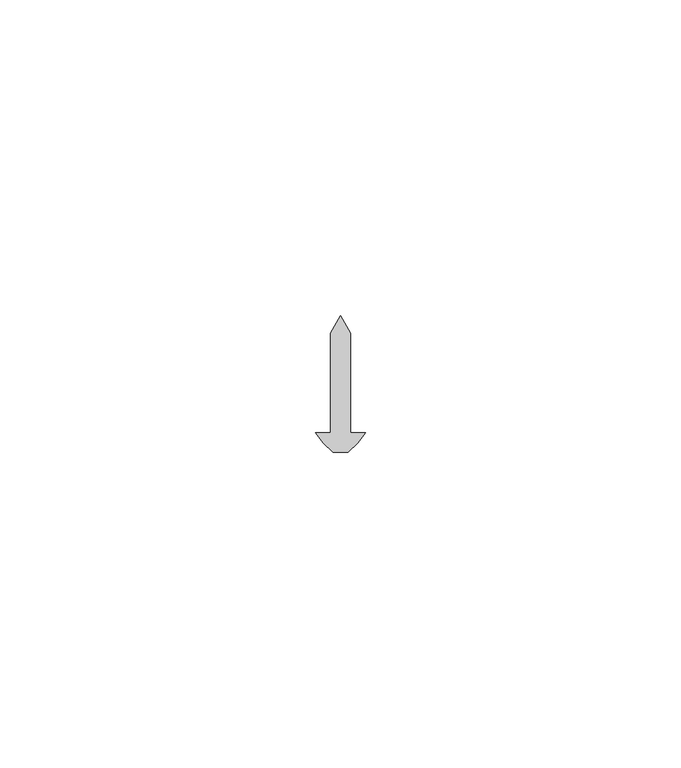
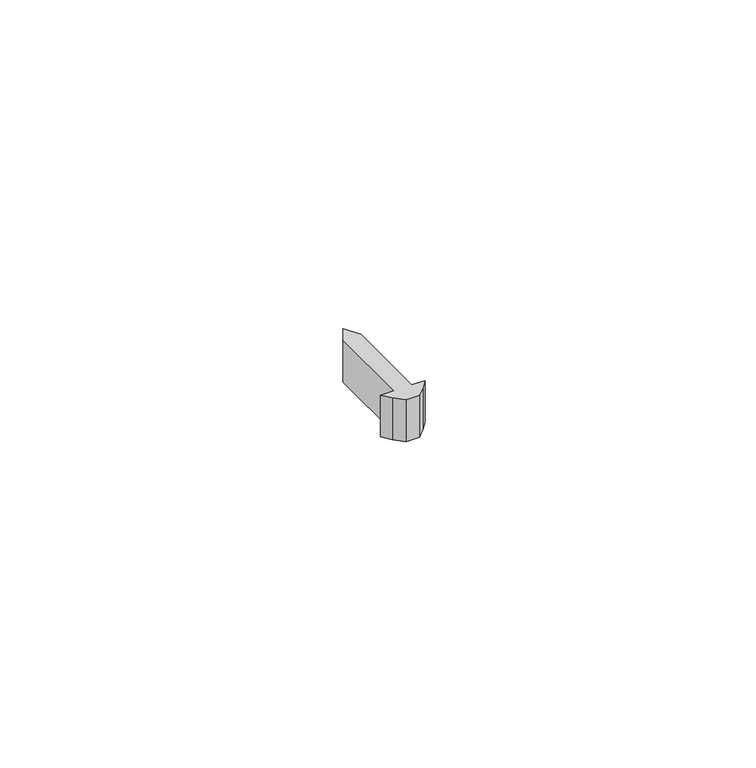
"""IFC4 building model written with IfcOpenShell, lengths in millimetres: proxy geometry, Generic Models 7:Generic Models 1:3:Generic Models 1:3 : Generic Models 7:Generic Models 1:305549:3:Generic Models 1:3:Generic Models 1:3 : Generic Models 7:Generic Models 1:305549:3 : Generic Models 7:Generic Models 1:3:Generic Models 1:3 : Generic Models 7:Generic Models 1:305549:301244:41 : Generic Models 7:Generic Models 1:3:Generic Models 1:3 : Generic Models 7:Generic Models 1:305549:3:Generic Models 1:3:Generic Models 1:3 : Generic Models 7:Generic Models 1:305549:3 : Generic Models 7:Generic Models 1:3:Generic Models 1:3 : Generic Models 7:Generic Models 1:305549:301244:308848."""

from ifc_helpers import new_model, si_unit, frame, origin, place, context, project, spatial, polyline, outline, extrude, source, transform, mapped, element, save


def generic_models_1cd3b07f(model_context):
    return source(origin(), model_context, "Body", "SweptSolid", [
        extrude(outline(polyline([(596149.4992239, -579084.8288841), (596149.4992239, -579069.0196286), (596151.0867239, -579066.2699979), (596152.6742239, -579069.0196286), (596152.6742239, -579084.8288841), (596155.0554739, -579084.8288841), (596153.8372784, -579086.3559421), (596152.2853882, -579087.9078323), (596149.8880597, -579087.9078323), (596148.3361695, -579086.3559421), (596147.1179739, -579084.8288841), (596149.4992239, -579084.8288841)])), frame((0.0, 0.0, 1237.45625), z_axis=(0.0, 0.0, 1.0), x_axis=(1.0, 0.0, 0.0)), (0.0, 0.0, 1.0), 7.9375),
    ])


if __name__ == "__main__":
    model = new_model("IFC4")
    model_context = context("Model", 3, world=origin())
    ifc_project = project(units=[si_unit("LENGTHUNIT", "METRE", prefix="MILLI")], contexts=[model_context])
    site = spatial("IfcSite", under=ifc_project)
    building = spatial("IfcBuilding", under=site)
    placement = place(None, origin())
    generic_models_shape = generic_models_1cd3b07f(model_context)
    element("IfcBuildingElementProxy", 1, Name="Generic Models 7:Generic Models 1:3:Generic Models 1:3 : Generic Models 7:Generic Models 1:305549:3:Generic Models 1:3:Generic Models 1:3 : Generic Models 7:Generic Models 1:305549:3 : Generic Models 7:Generic Models 1:3:Generic Models 1:3 : Generic Models 7:Generic Models 1:305549:301244:41 : Generic Models 7:Generic Models 1:3:Generic Models 1:3 : Generic Models 7:Generic Models 1:305549:3:Generic Models 1:3:Generic Models 1:3 : Generic Models 7:Generic Models 1:305549:3 : Generic Models 7:Generic Models 1:3:Generic Models 1:3 : Generic Models 7:Generic Models 1:305549:301244:308848", ObjectType="Generic Models 7:Generic Models 1:3:Generic Models 1:3 : Generic Models 7:Generic Models 1:305549:3:Generic Models 1:3:Generic Models 1:3 : Generic Models 7:Generic Models 1:305549:3 : Generic Models 7:Generic Models 1:3:Generic Models 1:3 : Generic Models 7:Generic Models 1:305549:301244:41 : Generic Models 7:Generic Models 1:3:Generic Models 1:3 : Generic Models 7:Generic Models 1:305549:3:Generic Models 1:3:Generic Models 1:3 : Generic Models 7:Generic Models 1:305549:3 : Generic Models 7:Generic Models 1:3:Generic Models 1:3 : Generic Models 7:Generic Models 1:305549:301244:308848", at=placement, inside=building, context=model_context, shape_type="MappedRepresentation", body=[
        mapped(generic_models_shape, transform((0.0, 0.0, 0.0), x_axis=(1.0, 0.0, 0.0), y_axis=(0.0, 1.0, 0.0), z_axis=(0.0, 0.0, 1.0))),
    ])
    save(model, "model.ifc")

# Revit data of these elements
# Type "Generic Models 7:Generic Models 1:3:Generic Models 1:3 : Generic Models 7:Generic Models 1:305549:3:Generic Models 1:3:Generic Models 1:3 : Generic Models 7:Generic Models 1:305549:3 : Generic Models 7:Generic Models 1:3:Generic Models 1:3 : Generic Models 7:Generic Models 1:305549:301244:41 : Generic Models 7:Generic Models 1:3:Generic Models 1:3 : Generic Models 7:Generic Models 1:305549:3:Generic Models 1:3:Generic Models 1:3 : Generic Models 7:Generic Models 1:305549:3 : Generic Models 7:Generic Models 1:3:Generic Models 1:3 : Generic Models 7:Generic Models 1:305549:301244:308848"
#   NameOverride = "Generic Models 7:Generic Models 1:3:Generic Models 1:3 : Generic Models 7:Generic Models 1:305549:3:Generic Models 1:3:Generic Models 1:3 : Generic Models 7:Generic Models 1:305549:3 : Generic Models 7:Generic Models 1:3:Generic Models 1:3 : Generic Models 7:Generic Models 1:305549:301244:308848"
#   ObjectTypeOverride = "Generic Models 1:3:Generic Models 1:3 : Generic Models 7:Generic Models 1:305549:3 : Generic Models 7:Generic Models 1:3:Generic Models 1:3 : Generic Models 7:Generic Models 1:305549:301244"
#   Reference = "Generic Models 1"
#   Tag = "308848"
# Element 1 (IfcBuildingElementProxy, "Generic Models 7:Generic Models 1:3:Generic Models 1:3 : Generic Models 7:Generic Models 1:305549:3:Generic Models 1:3:Generic Models 1:3 : Generic Models 7:Generic Models 1:305549:3 : Generic Models 7:Generic Models 1:3:Generic Models 1:3 : Generic Models 7:Generic Models 1:305549:301244:41 : Generic Models 7:Generic Models 1:3:Generic Models 1:3 : Generic Models 7:Generic Models 1:305549:3:Generic Models 1:3:Generic Models 1:3 : Generic Models 7:Generic Models 1:305549:3 : Generic Models 7:Generic Models 1:3:Generic Models 1:3 : Generic Models 7:Generic Models 1:305549:301244:308848")
#   Materials on its faces: "FASTENERS (T.B.D)"
# Materials
#   "FASTENERS (T.B.D)": class "Generic", colour RGB 120 120 120, transparency 0, Cost = 0
